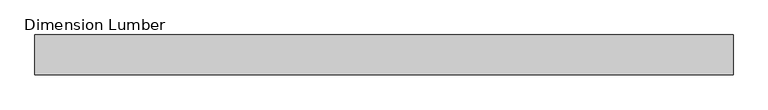
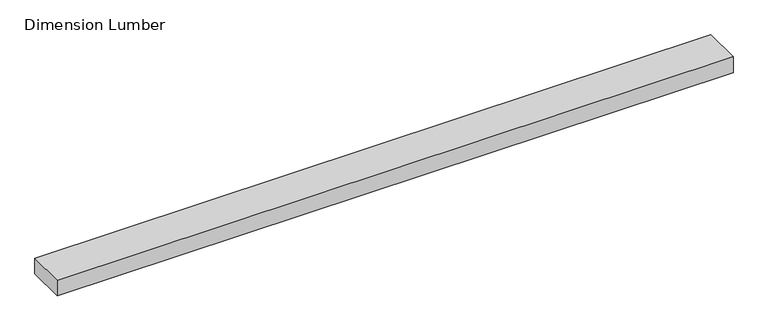
"""IFC4 building model written with IfcOpenShell, lengths in millimetres: beam geometry, Dimension Lumber : Opening Plate 2*4 Exterior."""

from ifc_helpers import new_model, si_unit, frame, origin, place, context, project, spatial, polyline, outline, extrude, source, transform, mapped, element, save


def dimension_lumber_8e7dc767(model_context):
    return source(origin(), model_context, "Body", "SweptSolid", [
        extrude(outline(polyline([(790.5750003, 44.45), (790.5750003, -44.45), (-771.5249997, -44.45), (-771.5249997, 44.45), (790.5750003, 44.45)])), frame((0.0, 0.0, -19.05), z_axis=(0.0, 0.0, 1.0), x_axis=(1.0, 0.0, 0.0)), (0.0, 0.0, 1.0), 38.1),
    ])


if __name__ == "__main__":
    model = new_model("IFC4")
    model_context = context("Model", 3, world=origin())
    ifc_project = project(units=[si_unit("LENGTHUNIT", "METRE", prefix="MILLI")], contexts=[model_context])
    site = spatial("IfcSite", under=ifc_project)
    building = spatial("IfcBuilding", under=site)
    placement = place(None, origin())
    dimension_lumber_shape = dimension_lumber_8e7dc767(model_context)
    element("IfcBeam", 1, ObjectType="Dimension Lumber : Opening Plate 2*4 Exterior", at=placement, inside=building, context=model_context, shape_type="MappedRepresentation", body=[
        mapped(dimension_lumber_shape, transform((0.0, 0.0, 0.0), x_axis=(1.0, 0.0, 0.0), y_axis=(0.0, 1.0, 0.0), z_axis=(0.0, 0.0, 1.0))),
    ])
    save(model, "model.ifc")

# Revit data of these elements
# Type "Dimension Lumber : Opening Plate 2*4 Exterior"
#   Assembly Code = "B10"
#   A = 0.0364583 SF
#   Length [instance default] = 5' - 0"
#   b = 0' - 3 1/2"
#   d = 0' - 1 1/2"
#   Structural Material [instance default] = Softwood, Lumber
# Element 1 (IfcBeam, "Dimension Lumber : Opening Plate 2*4 Exterior")
#   Structural Material = Douglas Fir #2
#   Materials on its faces: "Douglas Fir #2"
# Materials
#   "Softwood, Lumber": class "Wood", colour RGB 223 192 134, transparency 0, Description = "Pinus Echinata", Cost = 0
#   "Douglas Fir #2": class "Wood", colour RGB 223 192 134, transparency 0, Description = "Pinus Echinata", Cost = 0
